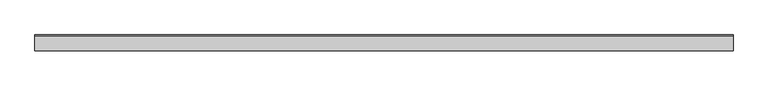
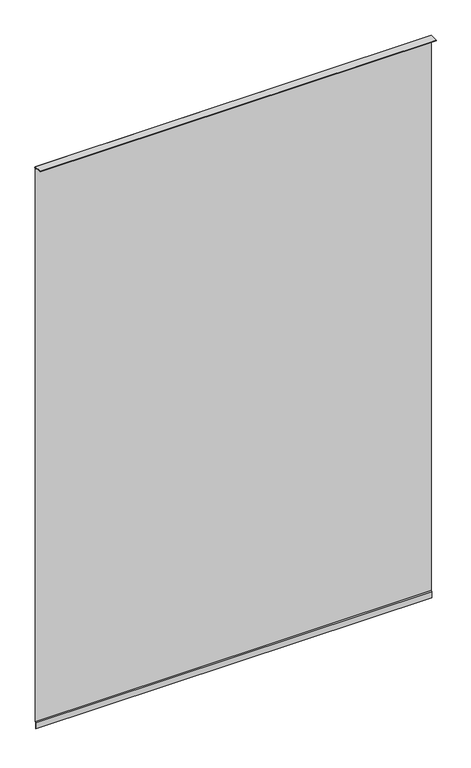
"""IFC4 building model written with IfcOpenShell, lengths in millimetres: proxy geometry, Generic Models 7:Generic Models 1:5:Generic Models 1:5 : Generic Models 7:Generic Models 1:337419:2 : Generic Models 7:Generic Models 1:5:Generic Models 1:5 : Generic Models 7:Generic Models 1:337419:311462."""

from ifc_helpers import new_model, si_unit, frame, origin, place, context, project, spatial, polyline, outline, extrude, source, transform, mapped, element, save


def generic_models_3737b989(model_context):
    return source(origin(), model_context, "Body", "SweptSolid", [
        extrude(outline(polyline([(-579014.8854955, 3723.8950904), (-579009.7444284, 3714.990501), (-579013.3913841, 3704.9705725), (-579013.3913841, 91.1977111), (-579017.0262729, 86.006552), (-579017.0262729, 46.3753703), (-579018.6137729, 46.3753703), (-579018.6137729, 86.5070888), (-579014.9788841, 91.698248), (-579014.9788841, 3705.2504916), (-579011.4893754, 3714.8378379), (-579015.7797318, 3722.2689531), (-579065.1919146, 3720.2101121), (-579065.2580031, 3721.7962359), (-579014.8854955, 3723.8950904)])), frame((593731.7367239, 0.0, 0.0), z_axis=(1.0, 0.0, 0.0), x_axis=(0.0, 1.0, 0.0)), (0.0, 0.0, 1.0), 2451.1),
    ])


if __name__ == "__main__":
    model = new_model("IFC4")
    model_context = context("Model", 3, world=origin())
    ifc_project = project(units=[si_unit("LENGTHUNIT", "METRE", prefix="MILLI")], contexts=[model_context])
    site = spatial("IfcSite", under=ifc_project)
    building = spatial("IfcBuilding", under=site)
    placement = place(None, origin())
    generic_models_shape = generic_models_3737b989(model_context)
    element("IfcBuildingElementProxy", 1, Name="Generic Models 7:Generic Models 1:5:Generic Models 1:5 : Generic Models 7:Generic Models 1:337419:2 : Generic Models 7:Generic Models 1:5:Generic Models 1:5 : Generic Models 7:Generic Models 1:337419:311462", ObjectType="Generic Models 7:Generic Models 1:5:Generic Models 1:5 : Generic Models 7:Generic Models 1:337419:2 : Generic Models 7:Generic Models 1:5:Generic Models 1:5 : Generic Models 7:Generic Models 1:337419:311462", at=placement, inside=building, context=model_context, shape_type="MappedRepresentation", body=[
        mapped(generic_models_shape, transform((0.0, 0.0, 0.0), x_axis=(1.0, 0.0, 0.0), y_axis=(0.0, 1.0, 0.0), z_axis=(0.0, 0.0, 1.0))),
    ])
    save(model, "model.ifc")

# Revit data of these elements
# Type "Generic Models 7:Generic Models 1:5:Generic Models 1:5 : Generic Models 7:Generic Models 1:337419:2 : Generic Models 7:Generic Models 1:5:Generic Models 1:5 : Generic Models 7:Generic Models 1:337419:311462"
#   NameOverride = "Generic Models 7:Generic Models 1:5:Generic Models 1:5 : Generic Models 7:Generic Models 1:337419:311462"
#   ObjectTypeOverride = "Generic Models 1:5 : Generic Models 7:Generic Models 1:337419"
#   Reference = "Generic Models 1"
#   Tag = "311462"
# Element 1 (IfcBuildingElementProxy, "Generic Models 7:Generic Models 1:5:Generic Models 1:5 : Generic Models 7:Generic Models 1:337419:2 : Generic Models 7:Generic Models 1:5:Generic Models 1:5 : Generic Models 7:Generic Models 1:337419:311462")
#   Materials on its faces: "UV STABLE WATER RESISTANT VAPOR PERMEABLE AIR BARRIER (WRB) - WRAP JAMBS/HEADERS - BLACK COLOR"
# Materials
#   "UV STABLE WATER RESISTANT VAPOR PERMEABLE AIR BARRIER (WRB) - WRAP JAMBS/HEADERS - BLACK COLOR": class "Generic", colour RGB 51 162 45, transparency 0, Description = "Polyethylene film membrane", Cost = 0
